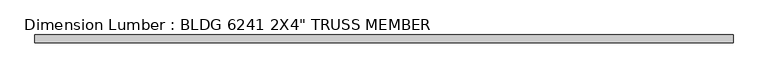
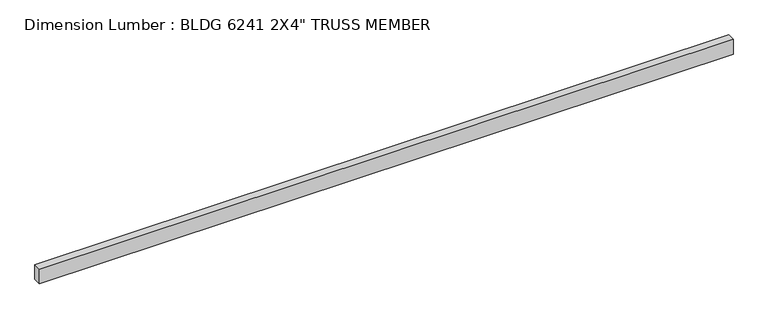
"""IFC4 building model written with IfcOpenShell, lengths in millimetres: beam geometry."""

import ifcopenshell
import ifcopenshell.guid

model = None  # the IFC model being written
_history = None  # IfcOwnerHistory: only IFC2X3 demands one
_inside = {}  # id of a spatial element -> (the spatial element, [elements in it])
_under = {}  # id of a project, library or spatial element -> (it, [spatial elements below it])
_declared = {}  # id of a project -> (the project, [libraries it declares])
_typed = {}  # id of a type object -> (the type object, [elements of that type])
_made_of = {}  # id of a material, layer set ... -> (it, [elements and type objects made of it])


def new_model(schema):
    """Start an empty IFC model of exactly this schema.

    Asked for "IFC4X3", IfcOpenShell would pick the latest addendum, in which some entities
    have other attributes; the version numbers below select the first issue.
    IFC2X3 requires an IfcOwnerHistory on every rooted entity: one is made here for all.
    """
    global model, _history
    if schema == "IFC4X3":
        model = ifcopenshell.file(schema_version=(4, 3, 0, 0))
    else:
        model = ifcopenshell.file(schema=schema)
    _inside.clear()
    _under.clear()
    _declared.clear()
    _typed.clear()
    _made_of.clear()
    _history = None
    if model.schema == "IFC2X3":
        org = make("IfcOrganization", Name="unknown")
        user = make(
            "IfcPersonAndOrganization",
            ThePerson=make("IfcPerson", FamilyName="unknown"),
            TheOrganization=org,
        )
        app = make(
            "IfcApplication",
            ApplicationDeveloper=org,
            Version="unknown",
            ApplicationFullName="unknown",
            ApplicationIdentifier="unknown",
        )
        _history = make(
            "IfcOwnerHistory",
            OwningUser=user,
            OwningApplication=app,
            ChangeAction="ADDED",
            CreationDate=0,
        )
    return model


def make(cls, **values):
    """One entity of the class cls with the attributes given. An attribute that is None is left unset."""
    return model.create_entity(
        cls, **{name: value for name, value in values.items() if value is not None}
    )


def rooted(cls, **values):
    """An entity with a GlobalId (a new one), such as an element, a storey or a relation."""
    return make(cls, GlobalId=ifcopenshell.guid.new(), OwnerHistory=_history, **values)


def si_unit(unit_type, name, prefix=None):
    """IfcSIUnit, for example si_unit("LENGTHUNIT", "METRE", prefix="MILLI")."""
    return make("IfcSIUnit", UnitType=unit_type, Prefix=prefix, Name=name)


def assignment(units):
    """IfcUnitAssignment: the units of a project."""
    return None if units is None else make("IfcUnitAssignment", Units=units)


def point(xyz):
    """IfcCartesianPoint."""
    return None if xyz is None else make("IfcCartesianPoint", Coordinates=xyz)


def direction(xyz):
    """IfcDirection."""
    return None if xyz is None else make("IfcDirection", DirectionRatios=xyz)


def frame(location, z_axis=None, x_axis=None):
    """IfcAxis2Placement3D, a coordinate frame: its origin and axes. An axis left out is left unset."""
    return make(
        "IfcAxis2Placement3D",
        Location=point(location),
        Axis=direction(z_axis),
        RefDirection=direction(x_axis),
    )


def origin():
    """The frame at (0, 0, 0) with its axes left unset."""
    return frame((0.0, 0.0, 0.0))


def place(relative_to, where):
    """IfcLocalPlacement: puts the frame where relative to a parent placement (None: the world)."""
    return make(
        "IfcLocalPlacement", PlacementRelTo=relative_to, RelativePlacement=where
    )


def context(
    kind, dimensions, precision=None, world=None, true_north=None, identifier=None
):
    """IfcGeometricRepresentationContext, for example the 3D "Model" context."""
    return make(
        "IfcGeometricRepresentationContext",
        ContextIdentifier=identifier,
        ContextType=kind,
        CoordinateSpaceDimension=dimensions,
        Precision=precision,
        WorldCoordinateSystem=world,
        TrueNorth=true_north,
    )


def project(units=None, contexts=None):
    """IfcProject with its units and contexts."""
    return rooted(
        "IfcProject",
        Name="project",
        RepresentationContexts=contexts,
        UnitsInContext=assignment(units),
    )


def spatial(cls, under=None, at=None, **own):
    """A site, building, storey or space (cls), placed at a placement, below another one or the project."""
    s = rooted(cls, ObjectPlacement=at, **own)
    if under is not None:
        _under.setdefault(under.id(), (under, []))[1].append(s)
    return s


def polyline(points):
    """IfcPolyline through the points."""
    return make("IfcPolyline", Points=[point(p) for p in points])


def outline(outer, holes=None, kind="AREA"):
    """IfcArbitraryClosedProfileDef: a profile drawn as a closed curve; with holes, ...WithVoids."""
    if holes is None:
        return make("IfcArbitraryClosedProfileDef", ProfileType=kind, OuterCurve=outer)
    return make(
        "IfcArbitraryProfileDefWithVoids",
        ProfileType=kind,
        OuterCurve=outer,
        InnerCurves=holes,
    )


def extrude(swept, where, along, depth):
    """IfcExtrudedAreaSolid: the profile swept, set in the frame where, extruded along a direction by depth."""
    return make(
        "IfcExtrudedAreaSolid",
        SweptArea=swept,
        Position=where,
        ExtrudedDirection=direction(along),
        Depth=depth,
    )


def shape(context_of_items, identifier, shape_type, items):
    """IfcShapeRepresentation: the items that make up one representation, for example the "Body"."""
    return make(
        "IfcShapeRepresentation",
        ContextOfItems=context_of_items,
        RepresentationIdentifier=identifier,
        RepresentationType=shape_type,
        Items=items,
    )


def source(mapping_origin, context_of_items, identifier, shape_type, items):
    """IfcRepresentationMap: a shape defined once, which mapped items show again and again."""
    return make(
        "IfcRepresentationMap",
        MappingOrigin=mapping_origin,
        MappedRepresentation=shape(context_of_items, identifier, shape_type, items),
    )


def transform(
    local_origin,
    x_axis=None,
    y_axis=None,
    z_axis=None,
    scale=None,
    scale2=None,
    scale3=None,
    uniform=True,
):
    """IfcCartesianTransformationOperator3D, or its non-uniform kind. x_axis, y_axis, z_axis: its Axis1, 2, 3."""
    if uniform:
        return make(
            "IfcCartesianTransformationOperator3D",
            Axis1=direction(x_axis),
            Axis2=direction(y_axis),
            LocalOrigin=point(local_origin),
            Scale=scale,
            Axis3=direction(z_axis),
        )
    return make(
        "IfcCartesianTransformationOperator3DnonUniform",
        Axis1=direction(x_axis),
        Axis2=direction(y_axis),
        LocalOrigin=point(local_origin),
        Scale=scale,
        Axis3=direction(z_axis),
        Scale2=scale2,
        Scale3=scale3,
    )


def mapped(mapping_source, mapping_target):
    """IfcMappedItem: shows the shape of a source again, moved by a transform."""
    return make(
        "IfcMappedItem", MappingSource=mapping_source, MappingTarget=mapping_target
    )


def made_of(thing, what):
    """Note that an element or type object is made of a material, layer set ...; save() writes the relation."""
    if what is not None:
        _made_of.setdefault(what.id(), (what, []))[1].append(thing)
    return thing


def element(
    cls,
    number,
    at=None,
    inside=None,
    cuts=None,
    type_object=None,
    material=None,
    context=None,
    identifier="Body",
    shape_type=None,
    held_by="IfcProductDefinitionShape",
    body=None,
    shapes=None,
    **own,
):
    """One element of the class cls, such as IfcWall. Its Tag is "e" and its number.

    at: its placement. inside: the storey or other place that contains it. cuts: it is an
    opening in that element (IfcRelVoidsElement). A single representation is given by context,
    identifier, shape_type and body (its items); several are given by shapes. held_by: the class
    of the entity that holds the representations. save() writes the other relations.
    """
    e = rooted(cls, Tag="e%d" % number, ObjectPlacement=at, **own)
    if body is not None:
        shapes = [shape(context, identifier, shape_type, body)]
    if shapes is not None:
        e.Representation = make(held_by, Representations=shapes)
    if inside is not None:
        _inside.setdefault(inside.id(), (inside, []))[1].append(e)
    if cuts is not None:
        rooted(
            "IfcRelVoidsElement", RelatingBuildingElement=cuts, RelatedOpeningElement=e
        )
    if type_object is not None:
        _typed.setdefault(type_object.id(), (type_object, []))[1].append(e)
    return made_of(e, material)


def aggregate(whole, parts):
    """IfcRelAggregates: a whole, such as a stair, and the parts it consists of."""
    return rooted("IfcRelAggregates", RelatingObject=whole, RelatedObjects=parts)


def save(model, path):
    """Write the relations noted so far, then the file.

    IfcRelAggregates (storeys below a building ...), IfcRelContainedInSpatialStructure (elements
    in a storey), IfcRelDefinesByType, IfcRelAssociatesMaterial and IfcRelDeclares: one each for
    every whole, place, type object, material and project.
    """
    for whole, parts in _under.values():
        aggregate(whole, parts)
    for where, things in _inside.values():
        rooted(
            "IfcRelContainedInSpatialStructure",
            RelatedElements=things,
            RelatingStructure=where,
        )
    for kind, things in _typed.values():
        rooted("IfcRelDefinesByType", RelatedObjects=things, RelatingType=kind)
    for what, things in _made_of.values():
        rooted("IfcRelAssociatesMaterial", RelatedObjects=things, RelatingMaterial=what)
    for by, libraries in _declared.values():
        rooted("IfcRelDeclares", RelatingContext=by, RelatedDefinitions=libraries)
    model.write(path)


def beam_175a3536(model_context):
    return source(origin(), model_context, "Body", "SweptSolid", [
        extrude(outline(polyline([(2249.4875, 25.4), (2249.4875, -25.4), (-2249.4874994, -25.4), (-2249.4874994, 25.4), (2249.4875, 25.4)])), frame((0.0, 0.0, -50.8), z_axis=(0.0, 0.0, 1.0), x_axis=(1.0, 0.0, 0.0)), (0.0, 0.0, 1.0), 101.6),
    ])


if __name__ == "__main__":
    model = new_model("IFC4")
    model_context = context("Model", 3, world=origin())
    ifc_project = project(units=[si_unit("LENGTHUNIT", "METRE", prefix="MILLI")], contexts=[model_context])
    site = spatial("IfcSite", under=ifc_project)
    building = spatial("IfcBuilding", under=site)
    placement = place(None, origin())
    beam_shape = beam_175a3536(model_context)
    element("IfcBeam", 1, ObjectType="Dimension Lumber : BLDG 6241 2X4\" TRUSS MEMBER", at=placement, inside=building, context=model_context, shape_type="MappedRepresentation", body=[
        mapped(beam_shape, transform((0.0, 0.0, 0.0), x_axis=(1.0, 0.0, 0.0), y_axis=(0.0, 1.0, 0.0), z_axis=(0.0, 0.0, 1.0))),
    ])
    save(model, "model.ifc")

# Revit data of these elements
# Type "Dimension Lumber : BLDG 6241 2X4\" TRUSS MEMBER"
#   Assembly Code = "B10"
#   A = 0.273472 SF
#   Length [instance default] = 5' - 0"
#   b = 0' - 2"
#   d = 0' - 4"
#   Structural Material [instance default] = Softwood, Lumber
# Element 1 (IfcBeam, "Dimension Lumber : BLDG 6241 2X4\" TRUSS MEMBER")
#   Materials on its faces: "Softwood, Lumber"
# Materials
#   "Softwood, Lumber": class "Wood", colour RGB 223 192 134, transparency 0, Description = "Pinus Echinata", Cost = 0
